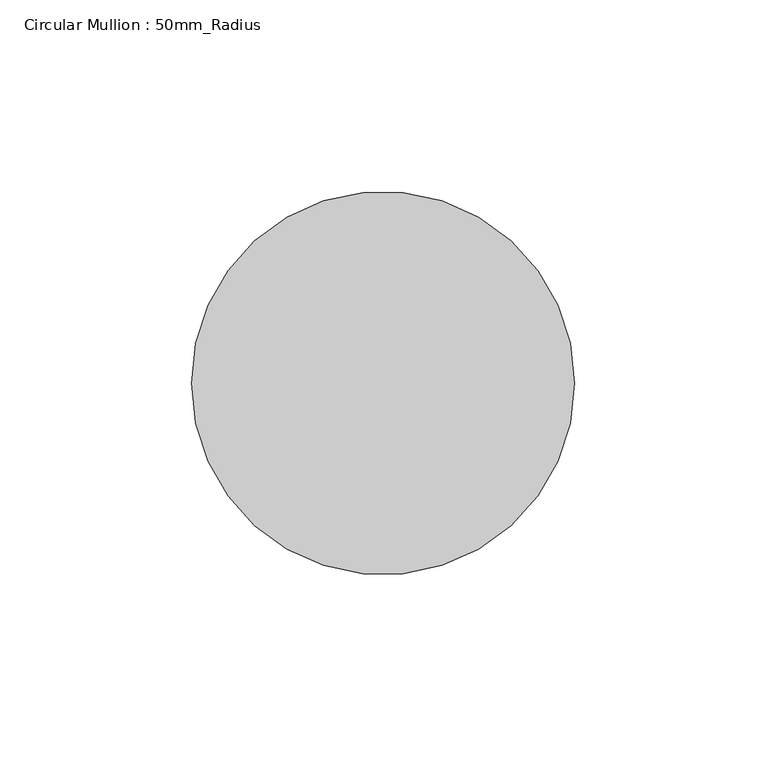
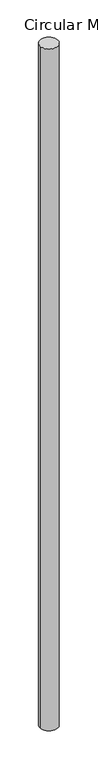
"""IFC4 building model written with IfcOpenShell, lengths in millimetres: member geometry, Circular Mullion : 50mm_Radius."""

from ifc_helpers import new_model, si_unit, point, frame, frame_2d, origin, place, context, project, spatial, circle_curve, trimmed, segment, composite_curve, outline, extrude, source, transform, mapped, element, save


def circular_mullion_50mm_radius_12d2e3e8(model_context):
    return source(origin(), model_context, "Body", "SweptSolid", [
        extrude(outline(composite_curve([segment(trimmed(circle_curve(frame_2d((-50.0, 0.0)), 50.0), [point((0.0, 0.0))], [point((-100.0, 0.0))], False, "CARTESIAN"), True, "CONTINUOUS"), segment(trimmed(circle_curve(frame_2d((-50.0, 0.0)), 50.0), [point((-100.0, 0.0))], [point((0.0, 0.0))], False, "CARTESIAN"), True, "CONTINUOUS")], self_intersect=False)), frame((0.0, 0.0, -4000.0), z_axis=(0.0, 0.0, 1.0), x_axis=(1.0, 0.0, 0.0)), (0.0, 0.0, 1.0), 4000.0),
    ])


if __name__ == "__main__":
    model = new_model("IFC4")
    model_context = context("Model", 3, world=origin())
    ifc_project = project(units=[si_unit("LENGTHUNIT", "METRE", prefix="MILLI")], contexts=[model_context])
    site = spatial("IfcSite", under=ifc_project)
    building = spatial("IfcBuilding", under=site)
    placement = place(None, origin())
    circular_mullion_50mm_radius_shape = circular_mullion_50mm_radius_12d2e3e8(model_context)
    element("IfcMember", 1, ObjectType="Circular Mullion : 50mm_Radius", at=placement, inside=building, context=model_context, shape_type="MappedRepresentation", body=[
        mapped(circular_mullion_50mm_radius_shape, transform((0.0, 0.0, 0.0), x_axis=(1.0, 0.0, 0.0), y_axis=(0.0, 1.0, 0.0), z_axis=(0.0, 0.0, 1.0))),
    ])
    save(model, "model.ifc")

# Revit data of these elements
# Type "Circular Mullion : 50mm_Radius"
#   Keynote = "H11"
#   built-in parameter 1007350 = 0.164042 (stored number, unit not read)
# Element 1 (IfcMember, "Circular Mullion : 50mm_Radius")
#   Materials on its faces: "Aluminium"
# Materials
#   "Aluminium": class "Metal", colour RGB 247 247 247, transparency 0, Description = "Aluminium 6061", Cost = 0
